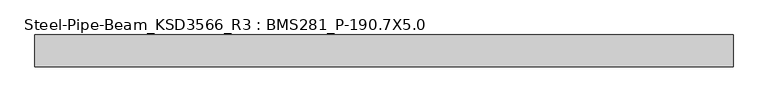
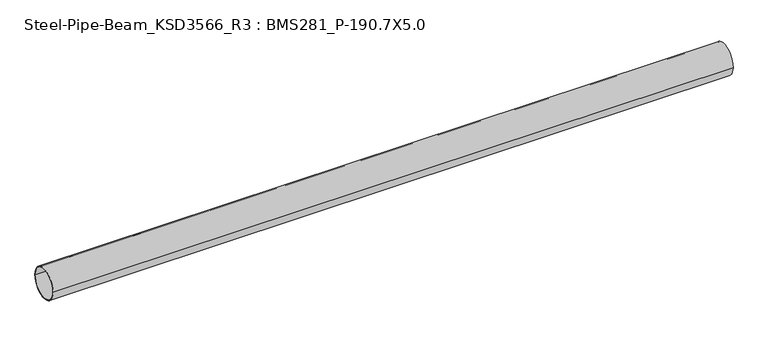
"""IFC4 building model written with IfcOpenShell, lengths in millimetres: member geometry, Steel-Pipe-Beam_KSD3566_R3 : BMS281_P-190.7X5.0."""

from ifc_helpers import new_model, si_unit, point, frame, origin, origin_2d, place, context, project, spatial, circle_curve, trimmed, segment, composite_curve, outline, extrude, source, transform, mapped, element, save


def steel_pipe_beam_ksd3566_r3_bms281_p_190_7x5_0_8d3283f1(model_context):
    return source(origin(), model_context, "Body", "SweptSolid", [
        extrude(outline(composite_curve([segment(trimmed(circle_curve(origin_2d(), 95.35), [point((-95.35, 0.0))], [point((95.35, 0.0))], False, "CARTESIAN"), True, "CONTINUOUS"), segment(trimmed(circle_curve(origin_2d(), 95.35), [point((95.35, 0.0))], [point((-95.35, 0.0))], False, "CARTESIAN"), True, "CONTINUOUS")], self_intersect=False), holes=[composite_curve([segment(trimmed(circle_curve(origin_2d(), 90.35), [point((90.35, 0.0))], [point((-90.35, 0.0))], True, "CARTESIAN"), True, "CONTINUOUS"), segment(trimmed(circle_curve(origin_2d(), 90.35), [point((-90.35, 0.0))], [point((90.35, 0.0))], True, "CARTESIAN"), True, "CONTINUOUS")], self_intersect=False)]), frame((-2106.2478846, 0.0, 0.0), z_axis=(1.0, 0.0, 0.0), x_axis=(0.0, 1.0, 0.0)), (0.0, 0.0, 1.0), 4152.3951135),
    ])


if __name__ == "__main__":
    model = new_model("IFC4")
    model_context = context("Model", 3, world=origin())
    ifc_project = project(units=[si_unit("LENGTHUNIT", "METRE", prefix="MILLI")], contexts=[model_context])
    site = spatial("IfcSite", under=ifc_project)
    building = spatial("IfcBuilding", under=site)
    placement = place(None, origin())
    steel_pipe_beam_ksd3566_r3_bms281_p_190_7x5_0_shape = steel_pipe_beam_ksd3566_r3_bms281_p_190_7x5_0_8d3283f1(model_context)
    element("IfcMember", 1, ObjectType="Steel-Pipe-Beam_KSD3566_R3 : BMS281_P-190.7X5.0", at=placement, inside=building, context=model_context, shape_type="MappedRepresentation", body=[
        mapped(steel_pipe_beam_ksd3566_r3_bms281_p_190_7x5_0_shape, transform((0.0, 0.0, 0.0), x_axis=(1.0, 0.0, 0.0), y_axis=(0.0, 1.0, 0.0), z_axis=(0.0, 0.0, 1.0))),
    ])
    save(model, "model.ifc")

# Revit data of these elements
# Type "Steel-Pipe-Beam_KSD3566_R3 : BMS281_P-190.7X5.0"
#   Keynote = "P-190.7X5.0"
#   SteelWeight = "Light"
#   t = 0.0050 m
#   Surface Area = 0.599102 m²/m
#   Section Area = 29.1697 cm²
#   Mass per Unit Length = 22.8982 kg/m
#   Length [instance default] = 1.5000 m
#   D = 0.1907 m
#   hec_material4 [instance default] = none
#   hec_material3 [instance default] = none
#   hec_material2 [instance default] = none
#   hec_material1 [instance default] = none
#   Structural Material [instance default] = Steel, 45-345
#   Assembly Code = ""
# Element 1 (IfcMember, "Steel-Pipe-Beam_KSD3566_R3 : BMS281_P-190.7X5.0")
#   Structural Material = none
# Materials
#   "Steel, 45-345": class "Metal", colour RGB 189 187 185, transparency 0, Description = "Steel 345 MPa", Cost = 0
